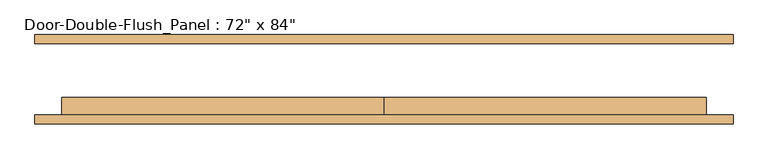
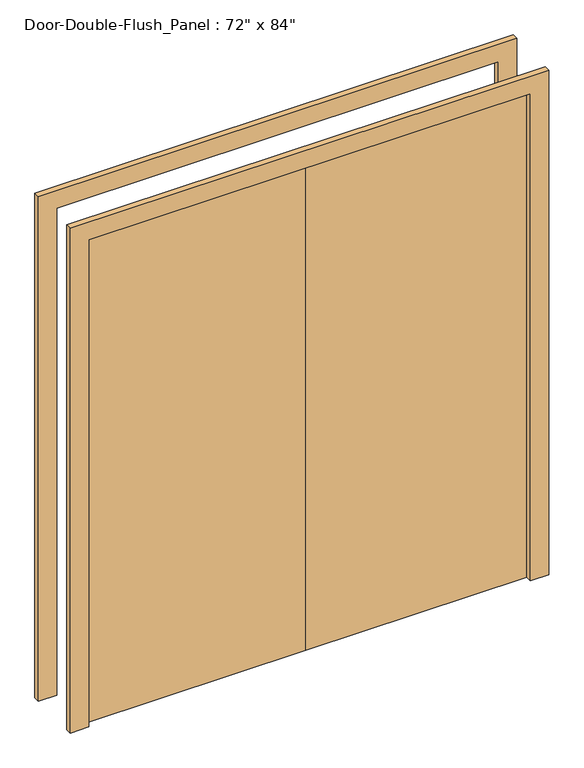
"""IFC4 building model written with IfcOpenShell, lengths in millimetres: door geometry."""

from ifc_helpers import new_model, si_unit, frame, origin, origin_with_axes, place, context, project, spatial, polyline, outline, extrude, source, transform, mapped, element, save


def door_51fa9bfd(model_context):
    return source(origin(), model_context, "Body", "SweptSolid", [
        extrude(outline(polyline([(2133.6, -914.4), (2133.6, 914.4), (0.0, 914.4), (0.0, 990.6), (2209.8, 990.6), (2209.8, -990.6), (0.0, -990.6), (0.0, -914.4), (2133.6, -914.4)])), frame((0.0, 101.6, 0.0), z_axis=(0.0, 1.0, 0.0), x_axis=(0.0, 0.0, 1.0)), (0.0, 0.0, 1.0), 25.4),
        extrude(outline(polyline([(2133.6, -914.4), (2133.6, 914.4), (0.0, 914.4), (0.0, 990.6), (2209.8, 990.6), (2209.8, -990.6), (0.0, -990.6), (0.0, -914.4), (2133.6, -914.4)])), frame((0.0, -127.0, 0.0), z_axis=(0.0, 1.0, 0.0), x_axis=(0.0, 0.0, 1.0)), (0.0, 0.0, 1.0), 25.4),
        extrude(outline(polyline([(0.0, -101.6), (0.0, -50.8), (914.4, -50.8), (914.4, -101.6), (0.0, -101.6)])), origin_with_axes(), (0.0, 0.0, 1.0), 2133.6),
        extrude(outline(polyline([(-914.4, -101.6), (-914.4, -50.8), (0.0, -50.8), (0.0, -101.6), (-914.4, -101.6)])), origin_with_axes(), (0.0, 0.0, 1.0), 2133.6),
    ])


if __name__ == "__main__":
    model = new_model("IFC4")
    model_context = context("Model", 3, world=origin())
    ifc_project = project(units=[si_unit("LENGTHUNIT", "METRE", prefix="MILLI")], contexts=[model_context])
    site = spatial("IfcSite", under=ifc_project)
    building = spatial("IfcBuilding", under=site)
    placement = place(None, origin())
    door_shape = door_51fa9bfd(model_context)
    element("IfcDoor", 1, ObjectType="Door-Double-Flush_Panel : 72\" x 84\"", at=placement, inside=building, context=model_context, shape_type="MappedRepresentation", body=[
        mapped(door_shape, transform((0.0, 0.0, 0.0), x_axis=(1.0, 0.0, 0.0), y_axis=(0.0, 1.0, 0.0), z_axis=(0.0, 0.0, 1.0))),
    ])
    save(model, "model.ifc")

# Revit data of these elements
# Type "Door-Double-Flush_Panel : 72\" x 84\""
#   Type Mark = "8"
#   Construction Type Id = "DOOR"
#   Assembly Code = "C1020"
#   Analytic Construction = "Wooden"
#   Thickness = 0' - 2"
#   Thermal Resistance (R) = 2.5876 (h·ft²·°F)/BTU
#   Swing Angle [instance default] = 90.00°
#   Panel Width = 3' - 0"
#   Heat Transfer Coefficient (U) = 0.3865 BTU/(h·ft²·°F)
#   Height = 7' - 0"
#   Trim Projection Ext = 0' - 1"
#   Trim Projection Int = 0' - 1"
#   Trim Width = 0' - 3"
#   Width = 6' - 0"
#   Define Thermal Properties by = 1
#   Define Thermal Properties by = 1
#   Panel Material = Wood - Birch - Solid Stained Light Low Gloss
#   Trim Material = Paint - Sienna
#   Visual Light Transmittance = 0
#   Solar Heat Gain Coefficient = 0
#   Function = (empty or 0)
#   Wall Closure = (empty or 0)
# Element 1 (IfcDoor, "Door-Double-Flush_Panel : 72\" x 84\"")
#   Materials on its faces: "Paint - Sienna", "Wood - Birch - Solid Stained Light Low Gloss"
# Materials
#   "Wood - Birch - Solid Stained Light Low Gloss": class "Wood", colour RGB 210 159 95, transparency 0, Cost = 0
#   "Paint - Sienna": class "Miscellaneous", colour RGB 118 70 51, transparency 0, Cost = 0
